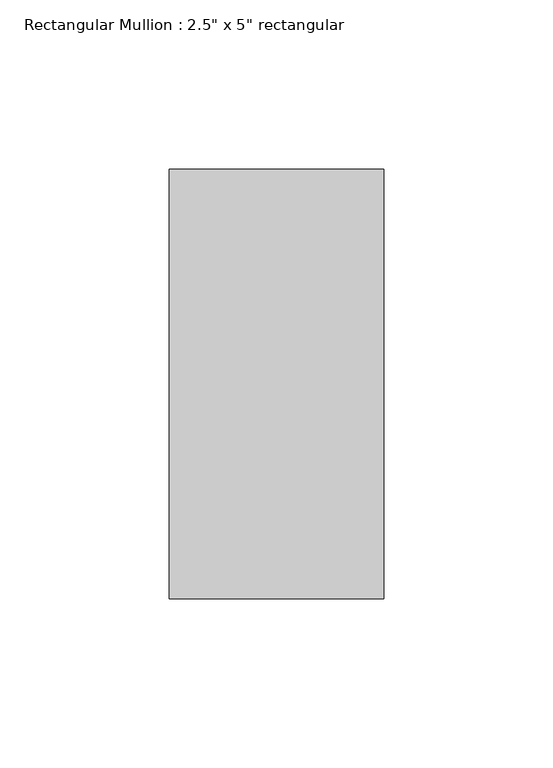
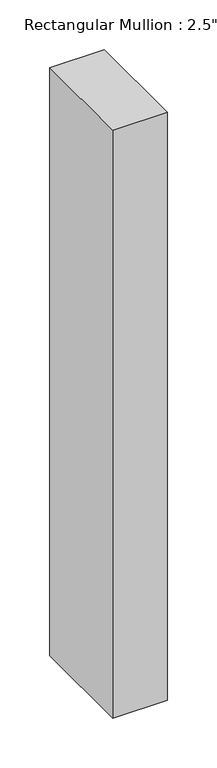
"""IFC4 building model written with IfcOpenShell, lengths in millimetres: member geometry."""

from ifc_helpers import new_model, si_unit, frame, origin, place, context, project, spatial, polyline, outline, extrude, source, transform, mapped, element, save


def member_a43dcf29(model_context):
    return source(origin(), model_context, "Body", "SweptSolid", [
        extrude(outline(polyline([(31.75, 63.5), (31.75, -63.5), (-31.75, -63.5), (-31.75, 63.5), (31.75, 63.5)])), frame((0.0, 0.0, -723.9), z_axis=(0.0, 0.0, 1.0), x_axis=(1.0, 0.0, 0.0)), (0.0, 0.0, 1.0), 723.9),
    ])


if __name__ == "__main__":
    model = new_model("IFC4")
    model_context = context("Model", 3, world=origin())
    ifc_project = project(units=[si_unit("LENGTHUNIT", "METRE", prefix="MILLI")], contexts=[model_context])
    site = spatial("IfcSite", under=ifc_project)
    building = spatial("IfcBuilding", under=site)
    placement = place(None, origin())
    member_shape = member_a43dcf29(model_context)
    element("IfcMember", 1, ObjectType="Rectangular Mullion : 2.5\" x 5\" rectangular", at=placement, inside=building, context=model_context, shape_type="MappedRepresentation", body=[
        mapped(member_shape, transform((0.0, 0.0, 0.0), x_axis=(1.0, 0.0, 0.0), y_axis=(0.0, 1.0, 0.0), z_axis=(0.0, 0.0, 1.0))),
    ])
    save(model, "model.ifc")

# Revit data of these elements
# Type "Rectangular Mullion : 2.5\" x 5\" rectangular"
#   built-in parameter 1007304 = 0.416667 (stored number, unit not read)
#   built-in parameter 1007301 = 0.104167 (stored number, unit not read)
#   built-in parameter 1007300 = 0.104167 (stored number, unit not read)
# Element 1 (IfcMember, "Rectangular Mullion : 2.5\" x 5\" rectangular")
#   Materials on its faces: "Aluminum"
# Materials
#   "Aluminum": class "Metal", colour RGB 247 247 247, transparency 0, Description = "Aluminum 6061", Cost = 0
